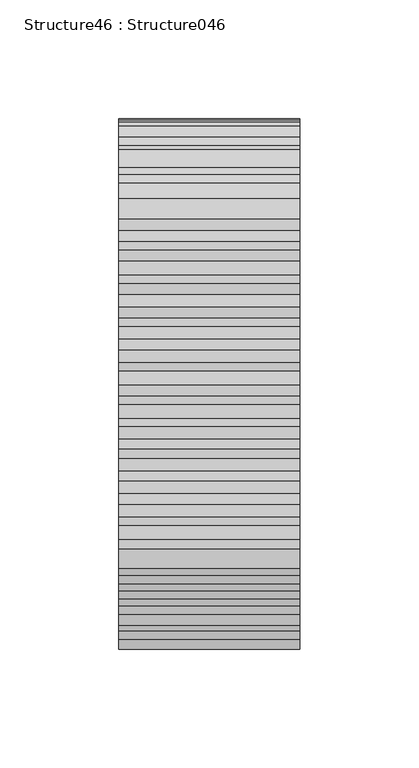
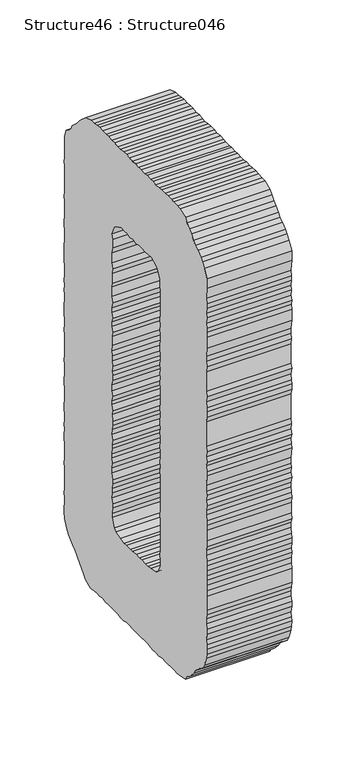
"""IFC4 building model written with IfcOpenShell, lengths in millimetres: proxy geometry, Structure46 : Structure046."""

from ifc_helpers import new_model, si_unit, frame, origin, place, context, project, spatial, polyline, outline, extrude, source, transform, mapped, element, save


def structure46_structure046_9ce00b97(model_context):
    return source(origin(), model_context, "Body", "SweptSolid", [
        extrude(outline(polyline([(255335.433373, 3554.0087015), (255333.0713952, 3558.1100706), (255328.3907639, 3561.025637), (255322.5291436, 3567.4857747), (255319.0086414, 3572.1423369), (255316.0882612, 3574.5107332), (255312.5677589, 3578.0103756), (255307.8871276, 3580.9532202), (255305.5476143, 3585.0706354), (255302.6272341, 3593.8285667), (255302.0255074, 3597.9540049), (255301.4462452, 3603.2122938), (255302.0255074, 3606.7295868), (255302.6272341, 3611.4134274), (255301.4462452, 3617.2718384), (255301.4462452, 3621.9813526), (255302.6272341, 3626.6571701), (255302.6272341, 3631.3410106), (255302.0255074, 3635.4407751), (255301.4462452, 3640.114988), (255301.4462452, 3653.6000842), (255302.0255074, 3658.3015753), (255302.0255074, 3663.5598643), (255301.4462452, 3668.8261762), (255302.0255074, 3672.3691429), (255301.4462452, 3677.6274319), (255301.4462452, 3682.3289231), (255302.0255074, 3686.4030139), (255302.6272341, 3691.6869765), (255302.6272341, 3696.3884676), (255301.4462452, 3700.4705815), (255302.0255074, 3705.7545441), (255302.0255074, 3715.7143242), (255301.4462452, 3720.9726131), (255302.0255074, 3725.0996559), (255302.6272341, 3730.3563402), (255302.6272341, 3734.47536), (255301.4462452, 3739.7416719), (255302.6272341, 3743.8414364), (255302.0255074, 3749.117376), (255302.6272341, 3752.6170184), (255302.6272341, 3758.485057), (255301.4462452, 3767.8607611), (255302.0255074, 3771.3860772), (255302.6272341, 3776.6427615), (255301.4462452, 3780.7441306), (255302.6272341, 3785.4456218), (255302.0255074, 3790.7039107), (255302.6272341, 3795.4037973), (255302.6272341, 3818.8310229), (255301.4462452, 3823.5341187), (255301.4462452, 3828.790803), (255302.0255074, 3832.3161191), (255302.6272341, 3837.6000817), (255301.4462452, 3843.432819), (255302.6272341, 3847.5598618), (255302.6272341, 3866.3032469), (255302.0255074, 3871.5599312), (255302.6272341, 3876.263027), (255302.6272341, 3880.9452629), (255301.4462452, 3889.1463965), (255301.4462452, 3899.7046941), (255302.0255074, 3904.3901392), (255301.4462452, 3908.46423), (255302.6272341, 3912.5896682), (255302.0255074, 3917.8479571), (255302.6272341, 3921.9733953), (255302.0255074, 3927.2332888), (255302.0255074, 3931.3346579), (255302.6272341, 3936.0345445), (255301.4462452, 3946.5511223), (255301.4462452, 3955.360401), (255305.5476143, 3962.9774586), (255309.0681165, 3967.0788276), (255311.4092345, 3969.994394), (255316.0882612, 3973.5197101), (255319.6103681, 3976.4368811), (255322.5291436, 3979.3781211), (255326.0512505, 3983.4794902), (255328.9700261, 3986.4046842), (255332.4905284, 3989.9460463), (255335.433373, 3993.4472933), (255343.6345066, 3996.390138), (255347.7342711, 3996.9645864), (255353.5958913, 3996.9645864), (255357.0955337, 3997.5486624), (255362.3762871, 3997.5486624), (255367.0569184, 3996.9645864), (255372.3392764, 3996.9645864), (255376.4390409, 3996.390138), (255381.6989344, 3996.390138), (255385.822768, 3996.9645864), (255389.9225325, 3996.390138), (255395.182426, 3996.9645864), (255398.7029283, 3996.390138), (255404.5645485, 3996.390138), (255408.0866554, 3996.9645864), (255412.7656821, 3997.5486624), (255418.6273023, 3996.390138), (255422.1478045, 3997.5486624), (255427.4076981, 3997.5486624), (255432.1107939, 3996.9645864), (255437.3915473, 3996.390138), (255440.8911897, 3996.390138), (255445.571821, 3997.5486624), (255450.8525744, 3996.390138), (255455.5332057, 3997.5486624), (255459.0537079, 3997.5486624), (255464.9153282, 3996.9645864), (255469.5959595, 3997.5486624), (255473.1164617, 3997.5486624), (255477.7970931, 3996.390138), (255482.5001888, 3996.390138), (255491.2805846, 3993.4472933), (255497.7214671, 3987.5792547), (255501.2419693, 3984.0635662), (255504.1832094, 3980.5623192), (255511.7842209, 3973.5197101), (255513.544472, 3969.418341), (255517.0649743, 3966.5043792), (255521.7456056, 3962.9774586), (255523.5058567, 3955.9348494), (255524.085119, 3950.6765605), (255524.085119, 3945.4182716), (255523.5058567, 3940.718385), (255523.5058567, 3936.6186205), (255524.6868456, 3931.9058971), (255524.085119, 3927.8077372), (255524.085119, 3923.1319197), (255523.5058567, 3918.4480792), (255523.5058567, 3913.1641166), (255524.085119, 3907.888177), (255523.5058567, 3903.2059411), (255524.6868456, 3899.1061766), (255523.5058567, 3894.4030808), (255523.5058567, 3879.7610648), (255524.6868456, 3875.686974), (255524.6868456, 3870.4030114), (255524.085119, 3866.8776953), (255524.085119, 3861.0192843), (255523.5058567, 3856.9179152), (255524.6868456, 3852.8181507), (255524.6868456, 3838.1761347), (255523.5058567, 3832.3161191), (255523.5058567, 3823.5341187), (255524.6868456, 3819.4150989), (255524.085119, 3813.5743386), (255524.6868456, 3810.0474179), (255524.085119, 3805.3459267), (255524.085119, 3800.6717138), (255524.6868456, 3795.960595), (255524.6868456, 3786.6298199), (255524.085119, 3781.9299333), (255524.085119, 3777.2444882), (255524.6868456, 3771.3860772), (255524.085119, 3767.2590344), (255524.085119, 3762.5848215), (255523.5058567, 3757.8753073), (255523.5058567, 3753.2171405), (255524.085119, 3747.9428055), (255524.6868456, 3743.2332913), (255523.5058567, 3739.1592005), (255523.5058567, 3730.3563402), (255524.6868456, 3725.0996559), (255524.6868456, 3720.9726131), (255524.085119, 3715.7143242), (255524.085119, 3705.1720727), (255524.6868456, 3701.0723082), (255524.6868456, 3696.3884676), (255524.085119, 3691.6869765), (255523.5058567, 3686.4030139), (255524.6868456, 3682.3289231), (255523.5058567, 3677.0449605), (255524.6868456, 3673.5276674), (255524.6868456, 3668.8261762), (255523.5058567, 3663.5598643), (255524.085119, 3659.4584952), (255524.085119, 3649.5003197), (255524.6868456, 3645.4262289), (255524.085119, 3640.7167147), (255524.085119, 3630.1824862), (255523.5058567, 3625.472972), (255523.5058567, 3621.3732075), (255524.6868456, 3616.69739), (255524.085119, 3612.5976255), (255523.5058567, 3607.8961343), (255524.6868456, 3603.2122938), (255524.6868456, 3597.9540049), (255524.085119, 3592.6700423), (255520.5646167, 3585.6274331), (255517.6442365, 3580.9532202), (255514.1237342, 3578.0103756), (255511.2033541, 3575.0851816), (255507.6828518, 3572.1423369), (255503.5814827, 3568.0682461), (255500.6627071, 3564.54293), (255494.1993602, 3558.1100706), (255491.2805846, 3554.0087015), (255483.0794511, 3551.0658569), (255477.7970931, 3551.6675836), (255473.1164617, 3552.242032), (255469.0166973, 3551.6675836), (255464.9153282, 3552.242032), (255459.6554346, 3551.6675836), (255455.5332057, 3551.6675836), (255449.6715855, 3552.242032), (255446.1735477, 3551.6675836), (255440.8911897, 3552.242032), (255436.7898206, 3551.0658569), (255432.1107939, 3551.0658569), (255427.4076981, 3552.242032), (255423.3079336, 3552.242032), (255418.0480401, 3551.6675836), (255403.9628218, 3551.6675836), (255399.3046549, 3552.242032), (255394.6031638, 3552.242032), (255389.9225325, 3551.0658569), (255385.822768, 3551.0658569), (255381.6989344, 3551.6675836), (255376.4390409, 3551.0658569), (255371.1582875, 3552.242032), (255367.0569184, 3551.6675836), (255362.3762871, 3551.6675836), (255357.0955337, 3552.242032), (255352.4149024, 3552.242032), (255348.3151379, 3551.6675836), (255344.2137688, 3552.242032), (255335.433373, 3554.0087015)]), holes=[polyline([(255443.8324297, 3918.4480792), (255435.6088317, 3922.5494483), (255430.929805, 3921.9733953), (255426.8284359, 3922.5494483), (255422.1478045, 3921.3748778), (255417.4463134, 3922.5494483), (255412.7656821, 3921.3748778), (255408.0866554, 3922.5494483), (255403.406024, 3922.5494483), (255398.123666, 3921.9733953), (255394.0239016, 3922.5494483), (255389.3208058, 3922.5494483), (255381.1421367, 3919.0321552), (255378.7801588, 3916.0909152), (255375.8597787, 3909.6468235), (255375.8597787, 3903.7884125), (255374.6787898, 3899.1061766), (255375.258052, 3895.0048075), (255374.6787898, 3889.7208449), (255374.6787898, 3875.686974), (255375.8597787, 3872.1440073), (255374.6787898, 3866.3032469), (255375.8597787, 3861.6178018), (255375.258052, 3858.1021133), (255374.6787898, 3852.2340747), (255375.8597787, 3848.1166595), (255375.8597787, 3844.0345457), (255374.6787898, 3838.1761347), (255374.6787898, 3834.0474873), (255375.8597787, 3828.790803), (255375.258052, 3824.1149855), (255375.8597787, 3820.5896694), (255375.258052, 3816.4883003), (255375.8597787, 3811.7884138), (255374.6787898, 3806.5317294), (255375.258052, 3801.2718359), (255375.258052, 3792.4705802), (255375.8597787, 3787.7867397), (255374.6787898, 3782.5027771), (255375.8597787, 3773.11905), (255374.6787898, 3768.4432325), (255375.8597787, 3764.9435901), (255375.258052, 3759.6596275), (255374.6787898, 3755.559863), (255375.8597787, 3750.8583719), (255375.258052, 3746.1745313), (255375.258052, 3740.3161203), (255375.8597787, 3736.7988273), (255374.6787898, 3732.1149867), (255375.8597787, 3726.8566978), (255375.258052, 3723.3313817), (255375.258052, 3713.3555556), (255374.6787898, 3708.6717151), (255374.6787898, 3703.4134261), (255375.258052, 3699.8881101), (255374.6787898, 3694.6298211), (255375.258052, 3689.9540036), (255375.8597787, 3685.8285655), (255374.6787898, 3681.1447249), (255375.258052, 3675.8687854), (255375.258052, 3667.0851803), (255374.6787898, 3662.3836892), (255375.258052, 3657.1254002), (255375.258052, 3651.8590883), (255375.8597787, 3648.3161216), (255374.6787898, 3643.0578326), (255375.258052, 3637.7995437), (255378.2008966, 3630.7392839), (255381.1421367, 3628.4158166), (255389.3208058, 3626.6571701), (255393.4221749, 3626.0554434), (255397.5219394, 3626.0554434), (255402.8042974, 3626.6571701), (255406.9040618, 3626.0554434), (255411.5846932, 3626.6571701), (255417.4463134, 3626.0554434), (255420.9668156, 3625.472972), (255426.8284359, 3626.0554434), (255430.929805, 3625.472972), (255436.2105583, 3626.6571701), (255443.8324297, 3628.4158166), (255446.1735477, 3630.7392839), (255449.0923232, 3638.9580681), (255449.0923232, 3643.0578326), (255448.513061, 3648.3161216), (255448.513061, 3652.4431643), (255449.6715855, 3657.1254002), (255449.0923232, 3662.3836892), (255449.0923232, 3666.5027089), (255448.513061, 3671.1849448), (255448.513061, 3675.2863139), (255449.6715855, 3681.1447249), (255449.6715855, 3685.8285655), (255449.0923232, 3690.512406), (255449.6715855, 3695.2122926), (255449.6715855, 3699.3136616), (255449.0923232, 3704.5879966), (255449.0923232, 3708.087639), (255448.513061, 3712.7971532), (255449.6715855, 3717.4729707), (255449.0923232, 3722.7312597), (255448.513061, 3726.8566978), (255448.513061, 3730.9323932), (255449.0923232, 3736.7988273), (255448.513061, 3740.9162424), (255449.6715855, 3746.1745313), (255449.6715855, 3749.701452), (255448.513061, 3754.3756649), (255449.6715855, 3759.0595054), (255449.6715855, 3764.9435901), (255448.513061, 3769.6274306), (255448.513061, 3774.3032481), (255449.0923232, 3777.8285642), (255448.513061, 3783.0868532), (255449.0923232, 3787.7867397), (255449.0923232, 3792.4705802), (255449.6715855, 3797.1463977), (255449.0923232, 3802.448011), (255449.0923232, 3811.2043377), (255448.513061, 3815.3313805), (255449.6715855, 3820.5896694), (255449.6715855, 3824.7167122), (255448.513061, 3828.790803), (255449.6715855, 3833.4730389), (255449.6715855, 3838.1761347), (255448.513061, 3843.432819), (255449.6715855, 3848.7167816), (255449.6715855, 3858.1021133), (255449.0923232, 3861.6178018), (255449.0923232, 3870.9790644), (255448.513061, 3875.686974), (255449.6715855, 3880.9452629), (255449.6715855, 3890.320967), (255448.513061, 3895.5888836), (255448.513061, 3903.7884125), (255449.6715855, 3908.46423), (255446.1735477, 3916.6653636), (255443.8324297, 3918.4480792)])]), frame((-38594.2176606, 0.0, 0.0), z_axis=(1.0, 0.0, 0.0), x_axis=(0.0, 1.0, 0.0)), (0.0, 0.0, 1.0), 76.2),
    ])


if __name__ == "__main__":
    model = new_model("IFC4")
    model_context = context("Model", 3, world=origin())
    ifc_project = project(units=[si_unit("LENGTHUNIT", "METRE", prefix="MILLI")], contexts=[model_context])
    site = spatial("IfcSite", under=ifc_project)
    building = spatial("IfcBuilding", under=site)
    placement = place(None, origin())
    structure46_structure046_shape = structure46_structure046_9ce00b97(model_context)
    element("IfcBuildingElementProxy", 1, Name="Structure46 : Structure046", ObjectType="Structure46 : Structure046", at=placement, inside=building, context=model_context, shape_type="MappedRepresentation", body=[
        mapped(structure46_structure046_shape, transform((0.0, 0.0, 0.0), x_axis=(1.0, 0.0, 0.0), y_axis=(0.0, 1.0, 0.0), z_axis=(0.0, 0.0, 1.0))),
    ])
    save(model, "model.ifc")

# Revit data of these elements
# Type "Structure46 : Structure046"
#   NameOverride = "Structure046"
# Element 1 (IfcBuildingElementProxy, "Structure46 : Structure046")
#   Materials on its faces: "BRUSHED ALUM. LETTERING"
# Materials
#   "BRUSHED ALUM. LETTERING": class "Unassigned", colour RGB 169 181 186, transparency 0, Cost = 0
